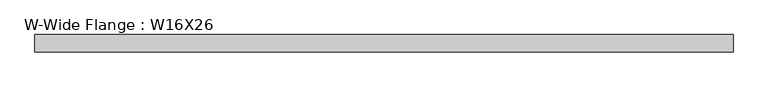
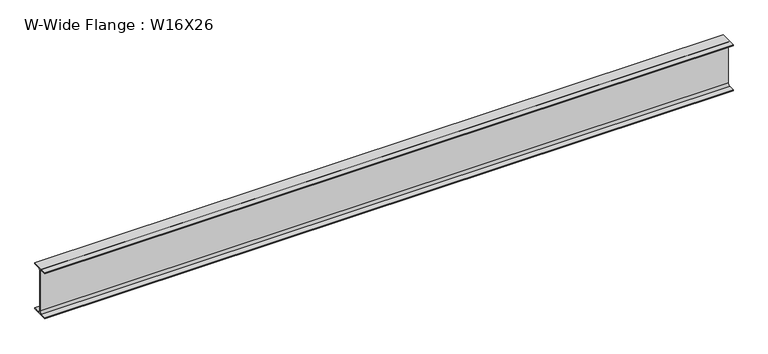
"""IFC4 building model written with IfcOpenShell, lengths in millimetres: beam geometry, W-Wide Flange : W16X26."""

from ifc_helpers import new_model, si_unit, point, frame, frame_2d, origin, place, context, project, spatial, polyline, circle_curve, trimmed, segment, composite_curve, outline, extrude, source, transform, mapped, element, save


def w_wide_flange_w16x26_d6617c16(model_context):
    return source(origin(), model_context, "Body", "SweptSolid", [
        extrude(outline(composite_curve([segment(polyline([(69.85, -190.627), (69.85, -199.39), (-69.85, -199.39), (-69.85, -190.627), (-21.3995, -190.627)]), True, "CONTINUOUS"), segment(trimmed(circle_curve(frame_2d((-21.3995, -172.4025)), 18.2245), [point((-21.3995, -190.627))], [point((-3.175, -172.4025))], True, "CARTESIAN"), True, "CONTINUOUS"), segment(polyline([(-3.175, -172.4025), (-3.175, 172.4025)]), True, "CONTINUOUS"), segment(trimmed(circle_curve(frame_2d((-21.3995, 172.4025)), 18.2245), [point((-3.175, 172.4025))], [point((-21.3995, 190.627))], True, "CARTESIAN"), True, "CONTINUOUS"), segment(polyline([(-21.3995, 190.627), (-69.85, 190.627), (-69.85, 199.39), (69.85, 199.39), (69.85, 190.627), (21.3995, 190.627)]), True, "CONTINUOUS"), segment(trimmed(circle_curve(frame_2d((21.3995, 172.4025)), 18.2245), [point((21.3995, 190.627))], [point((3.175, 172.4025))], True, "CARTESIAN"), True, "CONTINUOUS"), segment(polyline([(3.175, 172.4025), (3.175, -172.4025)]), True, "CONTINUOUS"), segment(trimmed(circle_curve(frame_2d((21.3995, -172.4025)), 18.2245), [point((3.175, -172.4025))], [point((21.3995, -190.627))], True, "CARTESIAN"), True, "CONTINUOUS"), segment(polyline([(21.3995, -190.627), (69.85, -190.627)]), True, "CONTINUOUS")], self_intersect=False)), frame((-2819.4, 0.0, 0.0), z_axis=(1.0, 0.0, 0.0), x_axis=(0.0, 1.0, 0.0)), (0.0, 0.0, 1.0), 5638.8),
    ])


if __name__ == "__main__":
    model = new_model("IFC4")
    model_context = context("Model", 3, world=origin())
    ifc_project = project(units=[si_unit("LENGTHUNIT", "METRE", prefix="MILLI")], contexts=[model_context])
    site = spatial("IfcSite", under=ifc_project)
    building = spatial("IfcBuilding", under=site)
    placement = place(None, origin())
    w_wide_flange_w16x26_shape = w_wide_flange_w16x26_d6617c16(model_context)
    element("IfcBeam", 1, ObjectType="W-Wide Flange : W16X26", at=placement, inside=building, context=model_context, shape_type="MappedRepresentation", body=[
        mapped(w_wide_flange_w16x26_shape, transform((0.0, 0.0, 0.0), x_axis=(1.0, 0.0, 0.0), y_axis=(0.0, 1.0, 0.0), z_axis=(0.0, 0.0, 1.0))),
    ])
    save(model, "model.ifc")

# Revit data of these elements
# Type "W-Wide Flange : W16X26"
#   Assembly Code = "B10"
#   W = 26
#   Length [instance default] = 5' - 0"
#   bf = 0' - 5 1/2"
#   d = 1' - 3.7"
#   k = 0' - 1 1/16"
#   k2 = 0' - 0.7175"
#   tf = 0' - 0.345"
#   tw = 0' - 0 1/4"
#   A = 0.0533333 SF
#   Structural Material [instance default] = Steel ASTM A992
# Element 1 (IfcBeam, "W-Wide Flange : W16X26")
#   Structural Material = Steel ASTM A36
#   Materials on its faces: "Steel ASTM A36"
# Materials
#   "Steel ASTM A992": class "Metal", colour RGB 199 199 199, transparency 0, Description = "Structural steel 50ksi", Cost = 0
#   "Steel ASTM A36": class "Metal", colour RGB 199 199 199, transparency 0, Description = "Structural steel, ASTM A36 Grade B, mill finish", Cost = 0
